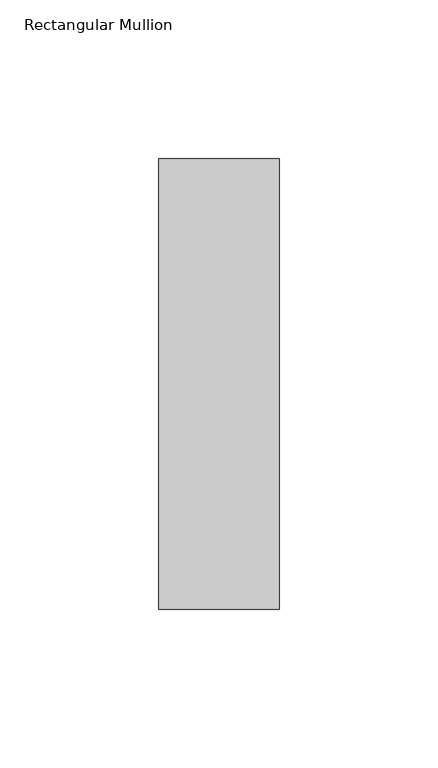
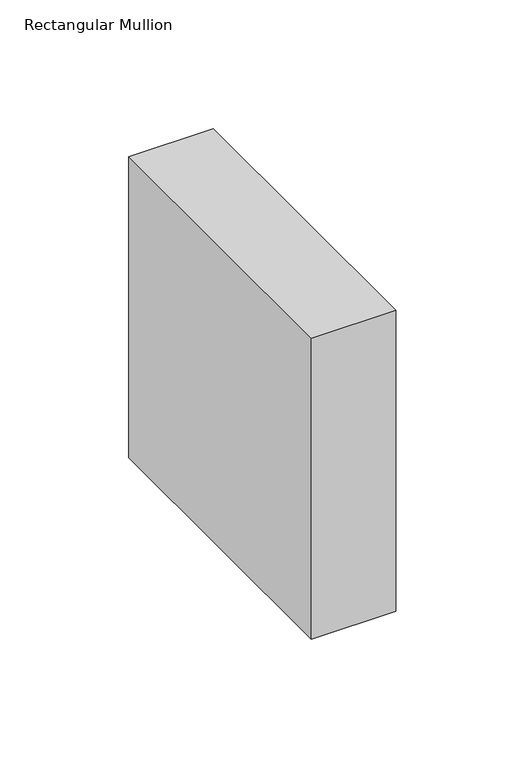
"""IFC4 building model written with IfcOpenShell, lengths in millimetres: member geometry, Rectangular Mullion : NLRS_21_CWM_hsb-regel 38x142_gen_rsf."""

from ifc_helpers import new_model, si_unit, frame, origin, place, context, project, spatial, polyline, outline, extrude, source, transform, mapped, element, save


def rectangular_mullion_9c2f1ecd(model_context):
    return source(origin(), model_context, "Body", "SweptSolid", [
        extrude(outline(polyline([(-38.0, -71.0), (-38.0, 71.0), (0.0, 71.0), (0.0, -71.0), (-38.0, -71.0)])), frame((0.0, 0.0, -142.9999997), z_axis=(0.0, 0.0, 1.0), x_axis=(1.0, 0.0, 0.0)), (0.0, 0.0, 1.0), 142.9999997),
    ])


if __name__ == "__main__":
    model = new_model("IFC4")
    model_context = context("Model", 3, world=origin())
    ifc_project = project(units=[si_unit("LENGTHUNIT", "METRE", prefix="MILLI")], contexts=[model_context])
    site = spatial("IfcSite", under=ifc_project)
    building = spatial("IfcBuilding", under=site)
    placement = place(None, origin())
    rectangular_mullion_shape = rectangular_mullion_9c2f1ecd(model_context)
    element("IfcMember", 1, ObjectType="Rectangular Mullion : NLRS_21_CWM_hsb-regel 38x142_gen_rsf", at=placement, inside=building, context=model_context, shape_type="MappedRepresentation", body=[
        mapped(rectangular_mullion_shape, transform((0.0, 0.0, 0.0), x_axis=(1.0, 0.0, 0.0), y_axis=(0.0, 1.0, 0.0), z_axis=(0.0, 0.0, 1.0))),
    ])
    save(model, "model.ifc")

# Revit data of these elements
# Type "Rectangular Mullion : NLRS_21_CWM_hsb-regel 38x142_gen_rsf"
#   Export Type to IFC As = "IfcWall"
#   Type IfcGUID = "07M7mRoiH1CR8m_RSKIwpF"
#   Assembly Code = "21.10"
#   built-in parameter 1007322 = 0.465879 (stored number, unit not read)
#   built-in parameter 1007321 = 0.062336 (stored number, unit not read)
#   built-in parameter 1007320 = 0.062336 (stored number, unit not read)
# Element 1 (IfcMember, "Rectangular Mullion : NLRS_21_CWM_hsb-regel 38x142_gen_rsf")
#   Materials on its faces: "NLRS_i2_hout naaldhout vuren_gen_rsf"
# Materials
#   "NLRS_i2_hout naaldhout vuren_gen_rsf": class "I - Hout", colour RGB 234 199 147, transparency 0, Keynote = "i2", Manufacturer = "Revit Standards Foundation", URL = "www.revitstandards.org", Description = "hout vuren", Cost = 0
